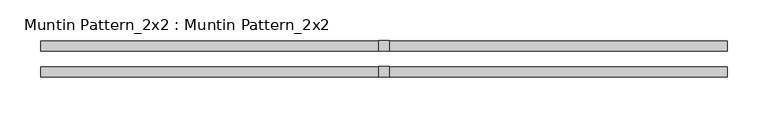
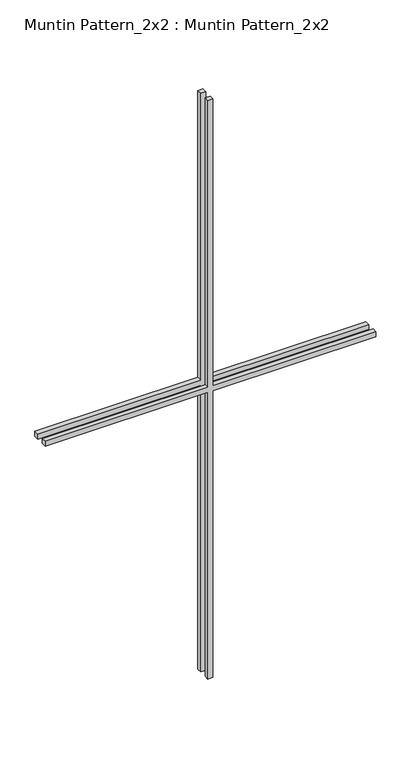
"""IFC4 building model written with IfcOpenShell, lengths in millimetres: proxy geometry, Muntin Pattern_2x2 : Muntin Pattern_2x2."""

from ifc_helpers import new_model, si_unit, frame, origin, place, context, project, spatial, polyline, outline, extrude, source, transform, mapped, element, save


def muntin_pattern_2x2_muntin_pattern_2x2_e2a5a0f5(model_context):
    return source(origin(), model_context, "Body", "SweptSolid", [
        extrude(outline(polyline([(781.05, -6.35), (781.05, -419.1), (768.35, -419.1), (768.35, -6.35), (0.0, -6.35), (0.0, 6.35), (768.35, 6.35), (768.35, 419.1), (781.05, 419.1), (781.05, 6.35), (1549.4, 6.35), (1549.4, -6.35), (781.05, -6.35)])), frame((0.0, 9.525, 0.0), z_axis=(0.0, 1.0, 0.0), x_axis=(0.0, 0.0, 1.0)), (0.0, 0.0, 1.0), 12.7),
        extrude(outline(polyline([(781.05, -6.35), (781.05, -419.1), (768.35, -419.1), (768.35, -6.35), (0.0, -6.35), (0.0, 6.35), (768.35, 6.35), (768.35, 419.1), (781.05, 419.1), (781.05, 6.35), (1549.4, 6.35), (1549.4, -6.35), (781.05, -6.35)])), frame((0.0, -22.225, 0.0), z_axis=(0.0, 1.0, 0.0), x_axis=(0.0, 0.0, 1.0)), (0.0, 0.0, 1.0), 12.7),
    ])


if __name__ == "__main__":
    model = new_model("IFC4")
    model_context = context("Model", 3, world=origin())
    ifc_project = project(units=[si_unit("LENGTHUNIT", "METRE", prefix="MILLI")], contexts=[model_context])
    site = spatial("IfcSite", under=ifc_project)
    building = spatial("IfcBuilding", under=site)
    placement = place(None, origin())
    muntin_pattern_2x2_muntin_pattern_2x2_shape = muntin_pattern_2x2_muntin_pattern_2x2_e2a5a0f5(model_context)
    element("IfcBuildingElementProxy", 1, Name="Muntin Pattern_2x2 : Muntin Pattern_2x2", ObjectType="Muntin Pattern_2x2 : Muntin Pattern_2x2", at=placement, inside=building, context=model_context, shape_type="MappedRepresentation", body=[
        mapped(muntin_pattern_2x2_muntin_pattern_2x2_shape, transform((0.0, 0.0, 0.0), x_axis=(1.0, 0.0, 0.0), y_axis=(0.0, 1.0, 0.0), z_axis=(0.0, 0.0, 1.0))),
    ])
    save(model, "model.ifc")

# Revit data of these elements
# Type "Muntin Pattern_2x2 : Muntin Pattern_2x2"
#   Width [instance default] = 4' - 0"
#   Thickness = 0' - 0 1/2"
#   Height [instance default] = 4' - 0"
#   Distance = 0' - 0 3/4"
#   Interior Material [instance default] = none
#   Exterior Material [instance default] = none
#   Default Elevation = 0
# Element 1 (IfcBuildingElementProxy, "Muntin Pattern_2x2 : Muntin Pattern_2x2")
#   Width = 2' - 9"
#   Height = 5' - 1"
#   Interior Material = Wood - Stained
#   Exterior Material = Clad - White
#   Materials on its faces: "Clad - White", "Wood - Stained"
# Materials
#   "Clad - White": class "Wood", colour RGB 242 242 238, transparency 0, Cost = 0
#   "Wood - Stained": class "Wood", colour RGB 224 178 126, transparency 0, Cost = 0
